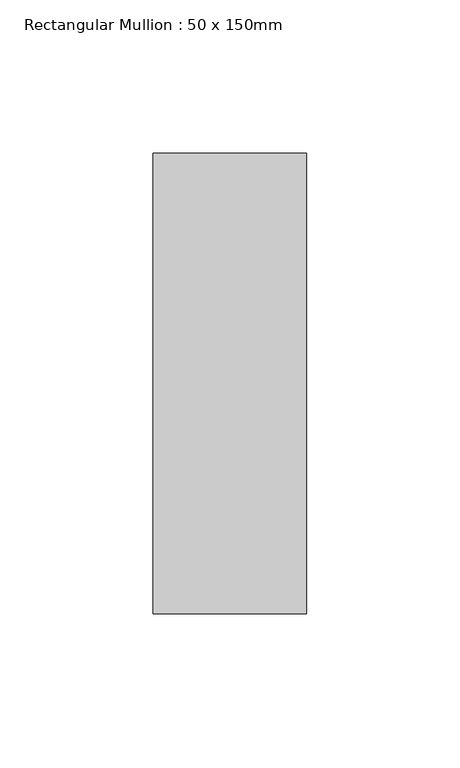
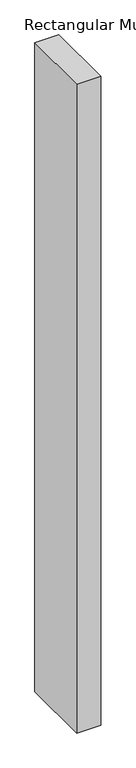
"""IFC4 building model written with IfcOpenShell, lengths in millimetres: member geometry, Rectangular Mullion : 50 x 150mm."""

from ifc_helpers import new_model, si_unit, frame, origin, place, context, project, spatial, polyline, outline, extrude, source, transform, mapped, element, save


def rectangular_mullion_50_x_150mm_4200193f(model_context):
    return source(origin(), model_context, "Body", "SweptSolid", [
        extrude(outline(polyline([(25.0, 75.0), (25.0, -75.0), (-25.0, -75.0), (-25.0, 75.0), (25.0, 75.0)])), frame((0.0, 0.0, -1425.0000001), z_axis=(0.0, 0.0, 1.0), x_axis=(1.0, 0.0, 0.0)), (0.0, 0.0, 1.0), 1425.0000001),
    ])


if __name__ == "__main__":
    model = new_model("IFC4")
    model_context = context("Model", 3, world=origin())
    ifc_project = project(units=[si_unit("LENGTHUNIT", "METRE", prefix="MILLI")], contexts=[model_context])
    site = spatial("IfcSite", under=ifc_project)
    building = spatial("IfcBuilding", under=site)
    placement = place(None, origin())
    rectangular_mullion_50_x_150mm_shape = rectangular_mullion_50_x_150mm_4200193f(model_context)
    element("IfcMember", 1, ObjectType="Rectangular Mullion : 50 x 150mm", at=placement, inside=building, context=model_context, shape_type="MappedRepresentation", body=[
        mapped(rectangular_mullion_50_x_150mm_shape, transform((0.0, 0.0, 0.0), x_axis=(1.0, 0.0, 0.0), y_axis=(0.0, 1.0, 0.0), z_axis=(0.0, 0.0, 1.0))),
    ])
    save(model, "model.ifc")

# Revit data of these elements
# Type "Rectangular Mullion : 50 x 150mm"
#   built-in parameter 1007304 = 0.492126 (stored number, unit not read)
#   built-in parameter 1007301 = 0.082021 (stored number, unit not read)
#   built-in parameter 1007300 = 0.082021 (stored number, unit not read)
# Element 1 (IfcMember, "Rectangular Mullion : 50 x 150mm")
#   Materials on its faces: "Aluminium"
# Materials
#   "Aluminium": class "Metal", colour RGB 247 247 247, transparency 0, Description = "Aluminium 6061", Cost = 0
